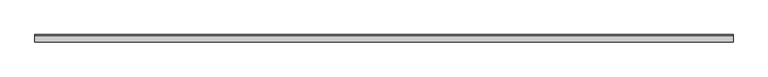
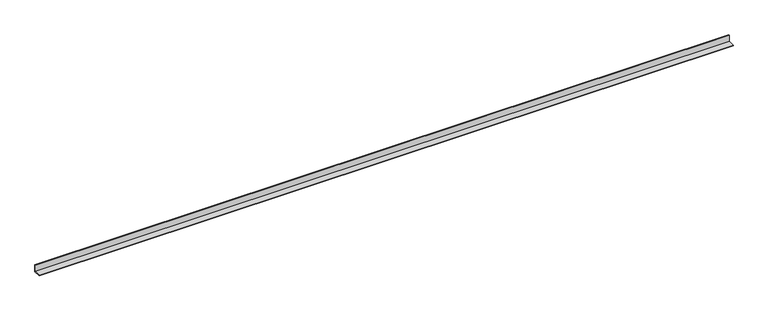
"""IFC4 building model written with IfcOpenShell, lengths in millimetres: proxy geometry, Generic Models 7:Generic Models 1:337419:Generic Models 1:337419 : Generic Models 7:Generic Models 1:337419:5 : Generic Models 7:Generic Models 1:337419:Generic Models 1:337419 : Generic Models 7:Generic Models 1:337419:301336."""

from ifc_helpers import new_model, si_unit, frame, origin, place, context, project, spatial, polyline, outline, extrude, source, transform, mapped, element, save


def generic_models_e5bd5cd4(model_context):
    return source(origin(), model_context, "Body", "SweptSolid", [
        extrude(outline(polyline([(-568199.3413841, 4843.5006), (-568250.1413841, 4843.5006), (-568250.1413841, 4848.2631), (-568204.1038841, 4848.2631), (-568204.1038841, 4894.3006), (-568199.3413841, 4894.3006), (-568199.3413841, 4843.5006)])), frame((597433.7867239, 0.0, 0.0), z_axis=(1.0, 0.0, 0.0), x_axis=(0.0, 1.0, 0.0)), (0.0, 0.0, 1.0), 4876.8),
    ])


if __name__ == "__main__":
    model = new_model("IFC4")
    model_context = context("Model", 3, world=origin())
    ifc_project = project(units=[si_unit("LENGTHUNIT", "METRE", prefix="MILLI")], contexts=[model_context])
    site = spatial("IfcSite", under=ifc_project)
    building = spatial("IfcBuilding", under=site)
    placement = place(None, origin())
    generic_models_shape = generic_models_e5bd5cd4(model_context)
    element("IfcBuildingElementProxy", 1, Name="Generic Models 7:Generic Models 1:337419:Generic Models 1:337419 : Generic Models 7:Generic Models 1:337419:5 : Generic Models 7:Generic Models 1:337419:Generic Models 1:337419 : Generic Models 7:Generic Models 1:337419:301336", ObjectType="Generic Models 7:Generic Models 1:337419:Generic Models 1:337419 : Generic Models 7:Generic Models 1:337419:5 : Generic Models 7:Generic Models 1:337419:Generic Models 1:337419 : Generic Models 7:Generic Models 1:337419:301336", at=placement, inside=building, context=model_context, shape_type="MappedRepresentation", body=[
        mapped(generic_models_shape, transform((0.0, 0.0, 0.0), x_axis=(1.0, 0.0, 0.0), y_axis=(0.0, 1.0, 0.0), z_axis=(0.0, 0.0, 1.0))),
    ])
    save(model, "model.ifc")

# Revit data of these elements
# Type "Generic Models 7:Generic Models 1:337419:Generic Models 1:337419 : Generic Models 7:Generic Models 1:337419:5 : Generic Models 7:Generic Models 1:337419:Generic Models 1:337419 : Generic Models 7:Generic Models 1:337419:301336"
#   NameOverride = "Generic Models 7:Generic Models 1:337419:Generic Models 1:337419 : Generic Models 7:Generic Models 1:337419:301336"
#   ObjectTypeOverride = "Generic Models 1:337419 : Generic Models 7:Generic Models 1:337419"
#   Reference = "Generic Models 1"
#   Tag = "301336"
# Element 1 (IfcBuildingElementProxy, "Generic Models 7:Generic Models 1:337419:Generic Models 1:337419 : Generic Models 7:Generic Models 1:337419:5 : Generic Models 7:Generic Models 1:337419:Generic Models 1:337419 : Generic Models 7:Generic Models 1:337419:301336")
#   Materials on its faces: "'ZEE' SECTION (8.0x3.5Z - SEE STRUCT. DWGS)"
# Materials
#   "'ZEE' SECTION (8.0x3.5Z - SEE STRUCT. DWGS)": class "Unassigned", colour RGB 210 209 208, transparency 0, Keynote = "M05121300.02", Cost = 0
